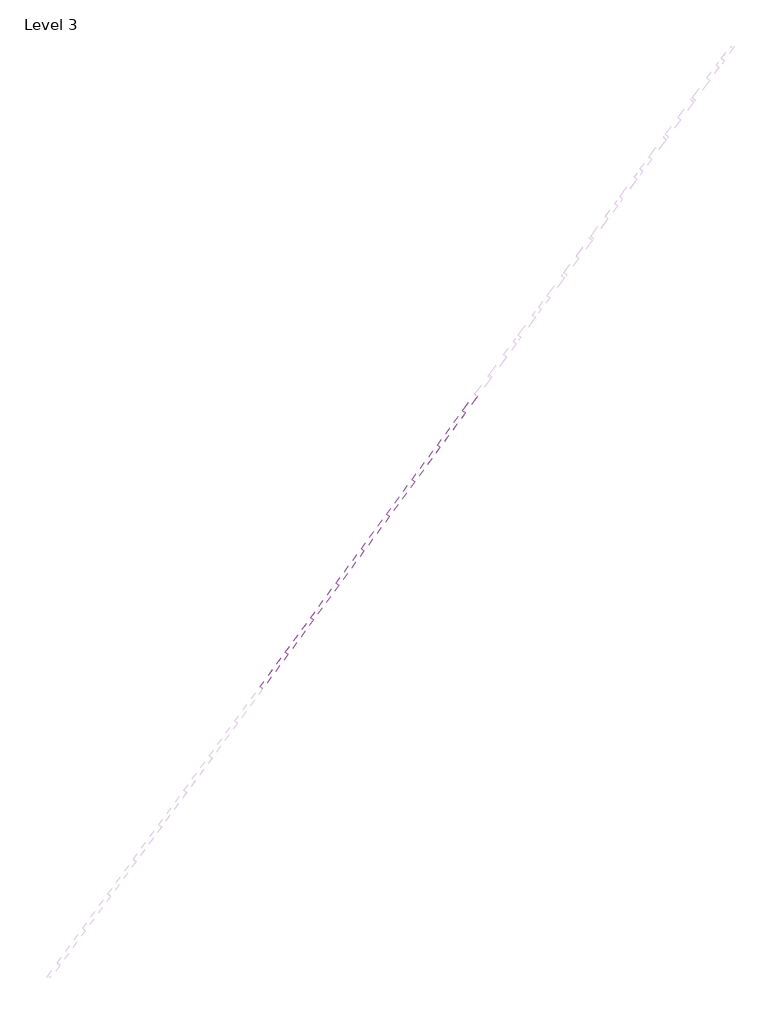
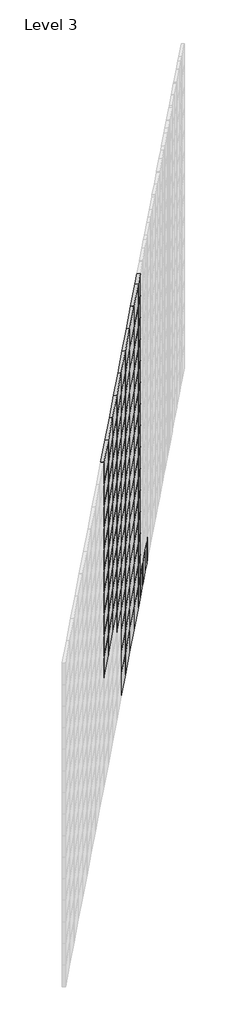
# One storey, part 3 of 9: 121 plates.
"""IFC4 building model written with IfcOpenShell, lengths in millimetres."""

import ifcopenshell
import ifcopenshell.guid

model = None  # the IFC model being written
_history = None  # IfcOwnerHistory: only IFC2X3 demands one
_inside = {}  # id of a spatial element -> (the spatial element, [elements in it])
_under = {}  # id of a project, library or spatial element -> (it, [spatial elements below it])
_declared = {}  # id of a project -> (the project, [libraries it declares])
_typed = {}  # id of a type object -> (the type object, [elements of that type])
_made_of = {}  # id of a material, layer set ... -> (it, [elements and type objects made of it])


def new_model(schema):
    """Start an empty IFC model of exactly this schema.

    Asked for "IFC4X3", IfcOpenShell would pick the latest addendum, in which some entities
    have other attributes; the version numbers below select the first issue.
    IFC2X3 requires an IfcOwnerHistory on every rooted entity: one is made here for all.
    """
    global model, _history
    if schema == "IFC4X3":
        model = ifcopenshell.file(schema_version=(4, 3, 0, 0))
    else:
        model = ifcopenshell.file(schema=schema)
    _inside.clear()
    _under.clear()
    _declared.clear()
    _typed.clear()
    _made_of.clear()
    _history = None
    if model.schema == "IFC2X3":
        org = make("IfcOrganization", Name="unknown")
        user = make(
            "IfcPersonAndOrganization",
            ThePerson=make("IfcPerson", FamilyName="unknown"),
            TheOrganization=org,
        )
        app = make(
            "IfcApplication",
            ApplicationDeveloper=org,
            Version="unknown",
            ApplicationFullName="unknown",
            ApplicationIdentifier="unknown",
        )
        _history = make(
            "IfcOwnerHistory",
            OwningUser=user,
            OwningApplication=app,
            ChangeAction="ADDED",
            CreationDate=0,
        )
    return model


def make(cls, **values):
    """One entity of the class cls with the attributes given. An attribute that is None is left unset."""
    return model.create_entity(
        cls, **{name: value for name, value in values.items() if value is not None}
    )


def rooted(cls, **values):
    """An entity with a GlobalId (a new one), such as an element, a storey or a relation."""
    return make(cls, GlobalId=ifcopenshell.guid.new(), OwnerHistory=_history, **values)


def si_unit(unit_type, name, prefix=None):
    """IfcSIUnit, for example si_unit("LENGTHUNIT", "METRE", prefix="MILLI")."""
    return make("IfcSIUnit", UnitType=unit_type, Prefix=prefix, Name=name)


def assignment(units):
    """IfcUnitAssignment: the units of a project."""
    return None if units is None else make("IfcUnitAssignment", Units=units)


def point(xyz):
    """IfcCartesianPoint."""
    return None if xyz is None else make("IfcCartesianPoint", Coordinates=xyz)


def direction(xyz):
    """IfcDirection."""
    return None if xyz is None else make("IfcDirection", DirectionRatios=xyz)


def frame(location, z_axis=None, x_axis=None):
    """IfcAxis2Placement3D, a coordinate frame: its origin and axes. An axis left out is left unset."""
    return make(
        "IfcAxis2Placement3D",
        Location=point(location),
        Axis=direction(z_axis),
        RefDirection=direction(x_axis),
    )


def origin():
    """The frame at (0, 0, 0) with its axes left unset."""
    return frame((0.0, 0.0, 0.0))


def origin_with_axes():
    """The frame at (0, 0, 0) with the z axis (0, 0, 1) and the x axis (1, 0, 0) written out."""
    return frame((0.0, 0.0, 0.0), z_axis=(0.0, 0.0, 1.0), x_axis=(1.0, 0.0, 0.0))


def place(relative_to, where):
    """IfcLocalPlacement: puts the frame where relative to a parent placement (None: the world)."""
    return make(
        "IfcLocalPlacement", PlacementRelTo=relative_to, RelativePlacement=where
    )


def context(
    kind, dimensions, precision=None, world=None, true_north=None, identifier=None
):
    """IfcGeometricRepresentationContext, for example the 3D "Model" context."""
    return make(
        "IfcGeometricRepresentationContext",
        ContextIdentifier=identifier,
        ContextType=kind,
        CoordinateSpaceDimension=dimensions,
        Precision=precision,
        WorldCoordinateSystem=world,
        TrueNorth=true_north,
    )


def project(units=None, contexts=None):
    """IfcProject with its units and contexts."""
    return rooted(
        "IfcProject",
        Name="project",
        RepresentationContexts=contexts,
        UnitsInContext=assignment(units),
    )


def spatial(cls, under=None, at=None, **own):
    """A site, building, storey or space (cls), placed at a placement, below another one or the project."""
    s = rooted(cls, ObjectPlacement=at, **own)
    if under is not None:
        _under.setdefault(under.id(), (under, []))[1].append(s)
    return s


def polyline(points):
    """IfcPolyline through the points."""
    return make("IfcPolyline", Points=[point(p) for p in points])


def outline(outer, holes=None, kind="AREA"):
    """IfcArbitraryClosedProfileDef: a profile drawn as a closed curve; with holes, ...WithVoids."""
    if holes is None:
        return make("IfcArbitraryClosedProfileDef", ProfileType=kind, OuterCurve=outer)
    return make(
        "IfcArbitraryProfileDefWithVoids",
        ProfileType=kind,
        OuterCurve=outer,
        InnerCurves=holes,
    )


def extrude(swept, where, along, depth):
    """IfcExtrudedAreaSolid: the profile swept, set in the frame where, extruded along a direction by depth."""
    return make(
        "IfcExtrudedAreaSolid",
        SweptArea=swept,
        Position=where,
        ExtrudedDirection=direction(along),
        Depth=depth,
    )


def shape(context_of_items, identifier, shape_type, items):
    """IfcShapeRepresentation: the items that make up one representation, for example the "Body"."""
    return make(
        "IfcShapeRepresentation",
        ContextOfItems=context_of_items,
        RepresentationIdentifier=identifier,
        RepresentationType=shape_type,
        Items=items,
    )


def source(mapping_origin, context_of_items, identifier, shape_type, items):
    """IfcRepresentationMap: a shape defined once, which mapped items show again and again."""
    return make(
        "IfcRepresentationMap",
        MappingOrigin=mapping_origin,
        MappedRepresentation=shape(context_of_items, identifier, shape_type, items),
    )


def transform(
    local_origin,
    x_axis=None,
    y_axis=None,
    z_axis=None,
    scale=None,
    scale2=None,
    scale3=None,
    uniform=True,
):
    """IfcCartesianTransformationOperator3D, or its non-uniform kind. x_axis, y_axis, z_axis: its Axis1, 2, 3."""
    if uniform:
        return make(
            "IfcCartesianTransformationOperator3D",
            Axis1=direction(x_axis),
            Axis2=direction(y_axis),
            LocalOrigin=point(local_origin),
            Scale=scale,
            Axis3=direction(z_axis),
        )
    return make(
        "IfcCartesianTransformationOperator3DnonUniform",
        Axis1=direction(x_axis),
        Axis2=direction(y_axis),
        LocalOrigin=point(local_origin),
        Scale=scale,
        Axis3=direction(z_axis),
        Scale2=scale2,
        Scale3=scale3,
    )


def mapped(mapping_source, mapping_target):
    """IfcMappedItem: shows the shape of a source again, moved by a transform."""
    return make(
        "IfcMappedItem", MappingSource=mapping_source, MappingTarget=mapping_target
    )


def made_of(thing, what):
    """Note that an element or type object is made of a material, layer set ...; save() writes the relation."""
    if what is not None:
        _made_of.setdefault(what.id(), (what, []))[1].append(thing)
    return thing


def element(
    cls,
    number,
    at=None,
    inside=None,
    cuts=None,
    type_object=None,
    material=None,
    context=None,
    identifier="Body",
    shape_type=None,
    held_by="IfcProductDefinitionShape",
    body=None,
    shapes=None,
    **own,
):
    """One element of the class cls, such as IfcWall. Its Tag is "e" and its number.

    at: its placement. inside: the storey or other place that contains it. cuts: it is an
    opening in that element (IfcRelVoidsElement). A single representation is given by context,
    identifier, shape_type and body (its items); several are given by shapes. held_by: the class
    of the entity that holds the representations. save() writes the other relations.
    """
    e = rooted(cls, Tag="e%d" % number, ObjectPlacement=at, **own)
    if body is not None:
        shapes = [shape(context, identifier, shape_type, body)]
    if shapes is not None:
        e.Representation = make(held_by, Representations=shapes)
    if inside is not None:
        _inside.setdefault(inside.id(), (inside, []))[1].append(e)
    if cuts is not None:
        rooted(
            "IfcRelVoidsElement", RelatingBuildingElement=cuts, RelatedOpeningElement=e
        )
    if type_object is not None:
        _typed.setdefault(type_object.id(), (type_object, []))[1].append(e)
    return made_of(e, material)


def aggregate(whole, parts):
    """IfcRelAggregates: a whole, such as a stair, and the parts it consists of."""
    return rooted("IfcRelAggregates", RelatingObject=whole, RelatedObjects=parts)


def save(model, path):
    """Write the relations noted so far, then the file.

    IfcRelAggregates (storeys below a building ...), IfcRelContainedInSpatialStructure (elements
    in a storey), IfcRelDefinesByType, IfcRelAssociatesMaterial and IfcRelDeclares: one each for
    every whole, place, type object, material and project.
    """
    for whole, parts in _under.values():
        aggregate(whole, parts)
    for where, things in _inside.values():
        rooted(
            "IfcRelContainedInSpatialStructure",
            RelatedElements=things,
            RelatingStructure=where,
        )
    for kind, things in _typed.values():
        rooted("IfcRelDefinesByType", RelatedObjects=things, RelatingType=kind)
    for what, things in _made_of.values():
        rooted("IfcRelAssociatesMaterial", RelatedObjects=things, RelatingMaterial=what)
    for by, libraries in _declared.values():
        rooted("IfcRelDeclares", RelatingContext=by, RelatedDefinitions=libraries)
    model.write(path)


def system_panel_glazed_2fc8f5ca(model_context):
    return source(origin(), model_context, "Body", "SweptSolid", [
        extrude(outline(polyline([(148.4832393, 24.5), (-148.4832393, 24.5), (-148.4832393, 49.5), (148.4832393, 49.5), (148.4832393, 24.5)])), origin_with_axes(), (0.0, 0.0, 1.0), 200.0),
    ])


def system_panel_glazed_b673c039(model_context):
    return source(origin(), model_context, "Body", "SweptSolid", [
        extrude(outline(polyline([(69.8854993, 24.5), (-69.8854993, 24.5), (-69.8854993, 49.5), (69.8854993, 49.5), (69.8854993, 24.5)])), origin_with_axes(), (0.0, 0.0, 1.0), 200.0),
    ])


def system_panel_glazed_de35cd91(model_context):
    return source(origin(), model_context, "Body", "SweptSolid", [
        extrude(outline(polyline([(6.4022601, 24.5), (-6.4022601, 24.5), (-6.4022601, 49.5), (6.4022601, 49.5), (6.4022601, 24.5)])), origin_with_axes(), (0.0, 0.0, 1.0), 200.0),
    ])


def system_panel_glazed_77252c6e(model_context):
    return source(origin(), model_context, "Body", "SweptSolid", [
        extrude(outline(polyline([(27.919021, 24.5), (-27.919021, 24.5), (-27.919021, 49.5), (27.919021, 49.5), (27.919021, 24.5)])), origin_with_axes(), (0.0, 0.0, 1.0), 200.0),
    ])


def system_panel_glazed_165eaad2(model_context):
    return source(origin(), model_context, "Body", "SweptSolid", [
        extrude(outline(polyline([(78.5977399, 24.5), (-78.5977399, 24.5), (-78.5977399, 49.5), (78.5977399, 49.5), (78.5977399, 24.5)])), origin_with_axes(), (0.0, 0.0, 1.0), 200.0),
    ])


def system_panel_glazed_1ea8d406(model_context):
    return source(origin(), model_context, "Body", "SweptSolid", [
        extrude(outline(polyline([(85.0, 24.5), (-85.0, 24.5), (-85.0, 49.5), (85.0, 49.5), (85.0, 24.5)])), origin_with_axes(), (0.0, 0.0, 1.0), 200.0),
    ])


def system_panel_glazed_41e93d41(model_context):
    return source(origin(), model_context, "Body", "SweptSolid", [
        extrude(outline(polyline([(57.080979, 24.5), (-57.080979, 24.5), (-57.080979, 49.5), (57.080979, 49.5), (57.080979, 24.5)])), origin_with_axes(), (0.0, 0.0, 1.0), 200.0),
    ])


model = new_model("IFC4")

# Units and contexts
model_context = context("Model", 3, world=origin())
ifc_project = project(units=[si_unit("LENGTHUNIT", "METRE", prefix="MILLI")], contexts=[model_context])

# Site, building, storey
site = spatial("IfcSite", under=ifc_project)
building = spatial("IfcBuilding", under=site)
storey = spatial("IfcBuildingStorey", under=building, Name="Level 3", Elevation=22950.0)

# Plates
placement = place(None, origin())
system_panel_glazed_shape = system_panel_glazed_2fc8f5ca(model_context)
element("IfcPlate", 1, ObjectType="System Panel : Glazed", at=placement, inside=storey, context=model_context, shape_type="MappedRepresentation", body=[
    mapped(system_panel_glazed_shape, transform((-34075.7749604, 27069.7374952, 35100.0), x_axis=(0.5920548138930122, 0.8058976965757569, 0.0), y_axis=(-0.8058976965757569, 0.5920548138930122, 0.0), z_axis=(0.0, 0.0, 1.0))),
])
element("IfcPlate", 2, ObjectType="System Panel : Glazed", at=placement, inside=storey, context=model_context, shape_type="MappedRepresentation", body=[
    mapped(system_panel_glazed_shape, transform((-33899.9545274, 27309.0620961, 35100.0), x_axis=(0.5920548138930122, 0.8058976965757569, 0.0), y_axis=(-0.8058976965757569, 0.5920548138930122, 0.0), z_axis=(0.0, 0.0, 1.0))),
])
element("IfcPlate", 3, ObjectType="System Panel : Glazed", at=placement, inside=storey, context=model_context, shape_type="MappedRepresentation", body=[
    mapped(system_panel_glazed_shape, transform((-33724.1340943, 27548.3866969, 35100.0), x_axis=(0.5920548138930122, 0.8058976965757569, 0.0), y_axis=(-0.8058976965757569, 0.5920548138930122, 0.0), z_axis=(0.0, 0.0, 1.0))),
])
element("IfcPlate", 4, ObjectType="System Panel : Glazed", at=placement, inside=storey, context=model_context, shape_type="MappedRepresentation", body=[
    mapped(system_panel_glazed_shape, transform((-33548.3136613, 27787.7112977, 35100.0), x_axis=(0.5920548138930122, 0.8058976965757569, 0.0), y_axis=(-0.8058976965757569, 0.5920548138930122, 0.0), z_axis=(0.0, 0.0, 1.0))),
])
element("IfcPlate", 5, ObjectType="System Panel : Glazed", at=placement, inside=storey, context=model_context, shape_type="MappedRepresentation", body=[
    mapped(system_panel_glazed_shape, transform((-34075.7749604, 27069.7374952, 35300.0), x_axis=(0.5920548138930122, 0.8058976965757569, 0.0), y_axis=(-0.8058976965757569, 0.5920548138930122, 0.0), z_axis=(0.0, 0.0, 1.0))),
])
element("IfcPlate", 6, ObjectType="System Panel : Glazed", at=placement, inside=storey, context=model_context, shape_type="MappedRepresentation", body=[
    mapped(system_panel_glazed_shape, transform((-33899.9545274, 27309.0620961, 35300.0), x_axis=(0.5920548138930122, 0.8058976965757569, 0.0), y_axis=(-0.8058976965757569, 0.5920548138930122, 0.0), z_axis=(0.0, 0.0, 1.0))),
])
element("IfcPlate", 7, ObjectType="System Panel : Glazed", at=placement, inside=storey, context=model_context, shape_type="MappedRepresentation", body=[
    mapped(system_panel_glazed_shape, transform((-33724.1340943, 27548.3866969, 35300.0), x_axis=(0.5920548138930122, 0.8058976965757569, 0.0), y_axis=(-0.8058976965757569, 0.5920548138930122, 0.0), z_axis=(0.0, 0.0, 1.0))),
])
element("IfcPlate", 8, ObjectType="System Panel : Glazed", at=placement, inside=storey, context=model_context, shape_type="MappedRepresentation", body=[
    mapped(system_panel_glazed_shape, transform((-33548.3136613, 27787.7112977, 35300.0), x_axis=(0.5920548138930122, 0.8058976965757569, 0.0), y_axis=(-0.8058976965757569, 0.5920548138930122, 0.0), z_axis=(0.0, 0.0, 1.0))),
])
element("IfcPlate", 9, ObjectType="System Panel : Glazed", at=placement, inside=storey, context=model_context, shape_type="MappedRepresentation", body=[
    mapped(system_panel_glazed_shape, transform((-34075.7749604, 27069.7374952, 35500.0), x_axis=(0.5920548138930122, 0.8058976965757569, 0.0), y_axis=(-0.8058976965757569, 0.5920548138930122, 0.0), z_axis=(0.0, 0.0, 1.0))),
])
element("IfcPlate", 10, ObjectType="System Panel : Glazed", at=placement, inside=storey, context=model_context, shape_type="MappedRepresentation", body=[
    mapped(system_panel_glazed_shape, transform((-33899.9545274, 27309.0620961, 35500.0), x_axis=(0.5920548138930122, 0.8058976965757569, 0.0), y_axis=(-0.8058976965757569, 0.5920548138930122, 0.0), z_axis=(0.0, 0.0, 1.0))),
])
element("IfcPlate", 11, ObjectType="System Panel : Glazed", at=placement, inside=storey, context=model_context, shape_type="MappedRepresentation", body=[
    mapped(system_panel_glazed_shape, transform((-33724.1340943, 27548.3866969, 35500.0), x_axis=(0.5920548138930122, 0.8058976965757569, 0.0), y_axis=(-0.8058976965757569, 0.5920548138930122, 0.0), z_axis=(0.0, 0.0, 1.0))),
])
element("IfcPlate", 12, ObjectType="System Panel : Glazed", at=placement, inside=storey, context=model_context, shape_type="MappedRepresentation", body=[
    mapped(system_panel_glazed_shape, transform((-33548.3136613, 27787.7112977, 35500.0), x_axis=(0.5920548138930122, 0.8058976965757569, 0.0), y_axis=(-0.8058976965757569, 0.5920548138930122, 0.0), z_axis=(0.0, 0.0, 1.0))),
])
element("IfcPlate", 13, ObjectType="System Panel : Glazed", at=placement, inside=storey, context=model_context, shape_type="MappedRepresentation", body=[
    mapped(system_panel_glazed_shape, transform((-34075.7749604, 27069.7374952, 35700.0), x_axis=(0.5920548138930122, 0.8058976965757569, 0.0), y_axis=(-0.8058976965757569, 0.5920548138930122, 0.0), z_axis=(0.0, 0.0, 1.0))),
])
element("IfcPlate", 14, ObjectType="System Panel : Glazed", at=placement, inside=storey, context=model_context, shape_type="MappedRepresentation", body=[
    mapped(system_panel_glazed_shape, transform((-33899.9545274, 27309.0620961, 35700.0), x_axis=(0.5920548138930122, 0.8058976965757569, 0.0), y_axis=(-0.8058976965757569, 0.5920548138930122, 0.0), z_axis=(0.0, 0.0, 1.0))),
])
element("IfcPlate", 15, ObjectType="System Panel : Glazed", at=placement, inside=storey, context=model_context, shape_type="MappedRepresentation", body=[
    mapped(system_panel_glazed_shape, transform((-33724.1340943, 27548.3866969, 35700.0), x_axis=(0.5920548138930122, 0.8058976965757569, 0.0), y_axis=(-0.8058976965757569, 0.5920548138930122, 0.0), z_axis=(0.0, 0.0, 1.0))),
])
element("IfcPlate", 16, ObjectType="System Panel : Glazed", at=placement, inside=storey, context=model_context, shape_type="MappedRepresentation", body=[
    mapped(system_panel_glazed_shape, transform((-33548.3136613, 27787.7112977, 35700.0), x_axis=(0.5920548138930122, 0.8058976965757569, 0.0), y_axis=(-0.8058976965757569, 0.5920548138930122, 0.0), z_axis=(0.0, 0.0, 1.0))),
])
element("IfcPlate", 17, ObjectType="System Panel : Glazed", at=placement, inside=storey, context=model_context, shape_type="MappedRepresentation", body=[
    mapped(system_panel_glazed_shape, transform((-34251.5953935, 26830.4128944, 35900.0), x_axis=(0.5920548138930122, 0.8058976965757569, 0.0), y_axis=(-0.8058976965757569, 0.5920548138930122, 0.0), z_axis=(0.0, 0.0, 1.0))),
])
element("IfcPlate", 18, ObjectType="System Panel : Glazed", at=placement, inside=storey, context=model_context, shape_type="MappedRepresentation", body=[
    mapped(system_panel_glazed_shape, transform((-34075.7749604, 27069.7374952, 35900.0), x_axis=(0.5920548138930122, 0.8058976965757569, 0.0), y_axis=(-0.8058976965757569, 0.5920548138930122, 0.0), z_axis=(0.0, 0.0, 1.0))),
])
element("IfcPlate", 19, ObjectType="System Panel : Glazed", at=placement, inside=storey, context=model_context, shape_type="MappedRepresentation", body=[
    mapped(system_panel_glazed_shape, transform((-33899.9545274, 27309.0620961, 35900.0), x_axis=(0.5920548138930122, 0.8058976965757569, 0.0), y_axis=(-0.8058976965757569, 0.5920548138930122, 0.0), z_axis=(0.0, 0.0, 1.0))),
])
element("IfcPlate", 20, ObjectType="System Panel : Glazed", at=placement, inside=storey, context=model_context, shape_type="MappedRepresentation", body=[
    mapped(system_panel_glazed_shape, transform((-33724.1340943, 27548.3866969, 35900.0), x_axis=(0.5920548138930122, 0.8058976965757569, 0.0), y_axis=(-0.8058976965757569, 0.5920548138930122, 0.0), z_axis=(0.0, 0.0, 1.0))),
])
element("IfcPlate", 21, ObjectType="System Panel : Glazed", at=placement, inside=storey, context=model_context, shape_type="MappedRepresentation", body=[
    mapped(system_panel_glazed_shape, transform((-33548.3136613, 27787.7112977, 35900.0), x_axis=(0.5920548138930122, 0.8058976965757569, 0.0), y_axis=(-0.8058976965757569, 0.5920548138930122, 0.0), z_axis=(0.0, 0.0, 1.0))),
])
element("IfcPlate", 22, ObjectType="System Panel : Glazed", at=placement, inside=storey, context=model_context, shape_type="MappedRepresentation", body=[
    mapped(system_panel_glazed_shape, transform((-34779.0566927, 26112.4390918, 36100.0), x_axis=(0.5920548138930122, 0.8058976965757569, 0.0), y_axis=(-0.8058976965757569, 0.5920548138930122, 0.0), z_axis=(0.0, 0.0, 1.0))),
])
element("IfcPlate", 23, ObjectType="System Panel : Glazed", at=placement, inside=storey, context=model_context, shape_type="MappedRepresentation", body=[
    mapped(system_panel_glazed_shape, transform((-34603.2362596, 26351.7636927, 36100.0), x_axis=(0.5920548138930122, 0.8058976965757569, 0.0), y_axis=(-0.8058976965757569, 0.5920548138930122, 0.0), z_axis=(0.0, 0.0, 1.0))),
])
element("IfcPlate", 24, ObjectType="System Panel : Glazed", at=placement, inside=storey, context=model_context, shape_type="MappedRepresentation", body=[
    mapped(system_panel_glazed_shape, transform((-34427.4158266, 26591.0882935, 36100.0), x_axis=(0.5920548138930122, 0.8058976965757569, 0.0), y_axis=(-0.8058976965757569, 0.5920548138930122, 0.0), z_axis=(0.0, 0.0, 1.0))),
])
element("IfcPlate", 25, ObjectType="System Panel : Glazed", at=placement, inside=storey, context=model_context, shape_type="MappedRepresentation", body=[
    mapped(system_panel_glazed_shape, transform((-34251.5953935, 26830.4128944, 36100.0), x_axis=(0.5920548138930122, 0.8058976965757569, 0.0), y_axis=(-0.8058976965757569, 0.5920548138930122, 0.0), z_axis=(0.0, 0.0, 1.0))),
])
element("IfcPlate", 26, ObjectType="System Panel : Glazed", at=placement, inside=storey, context=model_context, shape_type="MappedRepresentation", body=[
    mapped(system_panel_glazed_shape, transform((-34075.7749604, 27069.7374952, 36100.0), x_axis=(0.5920548138930122, 0.8058976965757569, 0.0), y_axis=(-0.8058976965757569, 0.5920548138930122, 0.0), z_axis=(0.0, 0.0, 1.0))),
])
element("IfcPlate", 27, ObjectType="System Panel : Glazed", at=placement, inside=storey, context=model_context, shape_type="MappedRepresentation", body=[
    mapped(system_panel_glazed_shape, transform((-33899.9545274, 27309.0620961, 36100.0), x_axis=(0.5920548138930122, 0.8058976965757569, 0.0), y_axis=(-0.8058976965757569, 0.5920548138930122, 0.0), z_axis=(0.0, 0.0, 1.0))),
])
element("IfcPlate", 28, ObjectType="System Panel : Glazed", at=placement, inside=storey, context=model_context, shape_type="MappedRepresentation", body=[
    mapped(system_panel_glazed_shape, transform((-33724.1340943, 27548.3866969, 36100.0), x_axis=(0.5920548138930122, 0.8058976965757569, 0.0), y_axis=(-0.8058976965757569, 0.5920548138930122, 0.0), z_axis=(0.0, 0.0, 1.0))),
])
element("IfcPlate", 29, ObjectType="System Panel : Glazed", at=placement, inside=storey, context=model_context, shape_type="MappedRepresentation", body=[
    mapped(system_panel_glazed_shape, transform((-33548.3136613, 27787.7112977, 36100.0), x_axis=(0.5920548138930122, 0.8058976965757569, 0.0), y_axis=(-0.8058976965757569, 0.5920548138930122, 0.0), z_axis=(0.0, 0.0, 1.0))),
])
element("IfcPlate", 30, ObjectType="System Panel : Glazed", at=placement, inside=storey, context=model_context, shape_type="MappedRepresentation", body=[
    mapped(system_panel_glazed_shape, transform((-34779.0566927, 26112.4390918, 36300.0), x_axis=(0.5920548138930122, 0.8058976965757569, 0.0), y_axis=(-0.8058976965757569, 0.5920548138930122, 0.0), z_axis=(0.0, 0.0, 1.0))),
])
element("IfcPlate", 31, ObjectType="System Panel : Glazed", at=placement, inside=storey, context=model_context, shape_type="MappedRepresentation", body=[
    mapped(system_panel_glazed_shape, transform((-34603.2362596, 26351.7636927, 36300.0), x_axis=(0.5920548138930122, 0.8058976965757569, 0.0), y_axis=(-0.8058976965757569, 0.5920548138930122, 0.0), z_axis=(0.0, 0.0, 1.0))),
])
element("IfcPlate", 32, ObjectType="System Panel : Glazed", at=placement, inside=storey, context=model_context, shape_type="MappedRepresentation", body=[
    mapped(system_panel_glazed_shape, transform((-34427.4158266, 26591.0882935, 36300.0), x_axis=(0.5920548138930122, 0.8058976965757569, 0.0), y_axis=(-0.8058976965757569, 0.5920548138930122, 0.0), z_axis=(0.0, 0.0, 1.0))),
])
element("IfcPlate", 33, ObjectType="System Panel : Glazed", at=placement, inside=storey, context=model_context, shape_type="MappedRepresentation", body=[
    mapped(system_panel_glazed_shape, transform((-34251.5953935, 26830.4128944, 36300.0), x_axis=(0.5920548138930122, 0.8058976965757569, 0.0), y_axis=(-0.8058976965757569, 0.5920548138930122, 0.0), z_axis=(0.0, 0.0, 1.0))),
])
element("IfcPlate", 34, ObjectType="System Panel : Glazed", at=placement, inside=storey, context=model_context, shape_type="MappedRepresentation", body=[
    mapped(system_panel_glazed_shape, transform((-34075.7749604, 27069.7374952, 36300.0), x_axis=(0.5920548138930122, 0.8058976965757569, 0.0), y_axis=(-0.8058976965757569, 0.5920548138930122, 0.0), z_axis=(0.0, 0.0, 1.0))),
])
element("IfcPlate", 35, ObjectType="System Panel : Glazed", at=placement, inside=storey, context=model_context, shape_type="MappedRepresentation", body=[
    mapped(system_panel_glazed_shape, transform((-33899.9545274, 27309.0620961, 36300.0), x_axis=(0.5920548138930122, 0.8058976965757569, 0.0), y_axis=(-0.8058976965757569, 0.5920548138930122, 0.0), z_axis=(0.0, 0.0, 1.0))),
])
element("IfcPlate", 36, ObjectType="System Panel : Glazed", at=placement, inside=storey, context=model_context, shape_type="MappedRepresentation", body=[
    mapped(system_panel_glazed_shape, transform((-33724.1340943, 27548.3866969, 36300.0), x_axis=(0.5920548138930122, 0.8058976965757569, 0.0), y_axis=(-0.8058976965757569, 0.5920548138930122, 0.0), z_axis=(0.0, 0.0, 1.0))),
])
element("IfcPlate", 37, ObjectType="System Panel : Glazed", at=placement, inside=storey, context=model_context, shape_type="MappedRepresentation", body=[
    mapped(system_panel_glazed_shape, transform((-33548.3136613, 27787.7112977, 36300.0), x_axis=(0.5920548138930122, 0.8058976965757569, 0.0), y_axis=(-0.8058976965757569, 0.5920548138930122, 0.0), z_axis=(0.0, 0.0, 1.0))),
])
element("IfcPlate", 38, ObjectType="System Panel : Glazed", at=placement, inside=storey, context=model_context, shape_type="MappedRepresentation", body=[
    mapped(system_panel_glazed_shape, transform((-34779.0566927, 26112.4390918, 36500.0), x_axis=(0.5920548138930122, 0.8058976965757569, 0.0), y_axis=(-0.8058976965757569, 0.5920548138930122, 0.0), z_axis=(0.0, 0.0, 1.0))),
])
element("IfcPlate", 39, ObjectType="System Panel : Glazed", at=placement, inside=storey, context=model_context, shape_type="MappedRepresentation", body=[
    mapped(system_panel_glazed_shape, transform((-34603.2362596, 26351.7636927, 36500.0), x_axis=(0.5920548138930122, 0.8058976965757569, 0.0), y_axis=(-0.8058976965757569, 0.5920548138930122, 0.0), z_axis=(0.0, 0.0, 1.0))),
])
element("IfcPlate", 40, ObjectType="System Panel : Glazed", at=placement, inside=storey, context=model_context, shape_type="MappedRepresentation", body=[
    mapped(system_panel_glazed_shape, transform((-34427.4158266, 26591.0882935, 36500.0), x_axis=(0.5920548138930122, 0.8058976965757569, 0.0), y_axis=(-0.8058976965757569, 0.5920548138930122, 0.0), z_axis=(0.0, 0.0, 1.0))),
])
element("IfcPlate", 41, ObjectType="System Panel : Glazed", at=placement, inside=storey, context=model_context, shape_type="MappedRepresentation", body=[
    mapped(system_panel_glazed_shape, transform((-34251.5953935, 26830.4128944, 36500.0), x_axis=(0.5920548138930122, 0.8058976965757569, 0.0), y_axis=(-0.8058976965757569, 0.5920548138930122, 0.0), z_axis=(0.0, 0.0, 1.0))),
])
element("IfcPlate", 42, ObjectType="System Panel : Glazed", at=placement, inside=storey, context=model_context, shape_type="MappedRepresentation", body=[
    mapped(system_panel_glazed_shape, transform((-34075.7749604, 27069.7374952, 36500.0), x_axis=(0.5920548138930122, 0.8058976965757569, 0.0), y_axis=(-0.8058976965757569, 0.5920548138930122, 0.0), z_axis=(0.0, 0.0, 1.0))),
])
element("IfcPlate", 43, ObjectType="System Panel : Glazed", at=placement, inside=storey, context=model_context, shape_type="MappedRepresentation", body=[
    mapped(system_panel_glazed_shape, transform((-33899.9545274, 27309.0620961, 36500.0), x_axis=(0.5920548138930122, 0.8058976965757569, 0.0), y_axis=(-0.8058976965757569, 0.5920548138930122, 0.0), z_axis=(0.0, 0.0, 1.0))),
])
element("IfcPlate", 44, ObjectType="System Panel : Glazed", at=placement, inside=storey, context=model_context, shape_type="MappedRepresentation", body=[
    mapped(system_panel_glazed_shape, transform((-33724.1340943, 27548.3866969, 36500.0), x_axis=(0.5920548138930122, 0.8058976965757569, 0.0), y_axis=(-0.8058976965757569, 0.5920548138930122, 0.0), z_axis=(0.0, 0.0, 1.0))),
])
element("IfcPlate", 45, ObjectType="System Panel : Glazed", at=placement, inside=storey, context=model_context, shape_type="MappedRepresentation", body=[
    mapped(system_panel_glazed_shape, transform((-33548.3136613, 27787.7112977, 36500.0), x_axis=(0.5920548138930122, 0.8058976965757569, 0.0), y_axis=(-0.8058976965757569, 0.5920548138930122, 0.0), z_axis=(0.0, 0.0, 1.0))),
])
element("IfcPlate", 46, ObjectType="System Panel : Glazed", at=placement, inside=storey, context=model_context, shape_type="MappedRepresentation", body=[
    mapped(system_panel_glazed_shape, transform((-34779.0566927, 26112.4390918, 36700.0), x_axis=(0.5920548138930122, 0.8058976965757569, 0.0), y_axis=(-0.8058976965757569, 0.5920548138930122, 0.0), z_axis=(0.0, 0.0, 1.0))),
])
element("IfcPlate", 47, ObjectType="System Panel : Glazed", at=placement, inside=storey, context=model_context, shape_type="MappedRepresentation", body=[
    mapped(system_panel_glazed_shape, transform((-34603.2362596, 26351.7636927, 36700.0), x_axis=(0.5920548138930122, 0.8058976965757569, 0.0), y_axis=(-0.8058976965757569, 0.5920548138930122, 0.0), z_axis=(0.0, 0.0, 1.0))),
])
element("IfcPlate", 48, ObjectType="System Panel : Glazed", at=placement, inside=storey, context=model_context, shape_type="MappedRepresentation", body=[
    mapped(system_panel_glazed_shape, transform((-34427.4158266, 26591.0882935, 36700.0), x_axis=(0.5920548138930122, 0.8058976965757569, 0.0), y_axis=(-0.8058976965757569, 0.5920548138930122, 0.0), z_axis=(0.0, 0.0, 1.0))),
])
element("IfcPlate", 49, ObjectType="System Panel : Glazed", at=placement, inside=storey, context=model_context, shape_type="MappedRepresentation", body=[
    mapped(system_panel_glazed_shape, transform((-34251.5953935, 26830.4128944, 36700.0), x_axis=(0.5920548138930122, 0.8058976965757569, 0.0), y_axis=(-0.8058976965757569, 0.5920548138930122, 0.0), z_axis=(0.0, 0.0, 1.0))),
])
element("IfcPlate", 50, ObjectType="System Panel : Glazed", at=placement, inside=storey, context=model_context, shape_type="MappedRepresentation", body=[
    mapped(system_panel_glazed_shape, transform((-34075.7749604, 27069.7374952, 36700.0), x_axis=(0.5920548138930122, 0.8058976965757569, 0.0), y_axis=(-0.8058976965757569, 0.5920548138930122, 0.0), z_axis=(0.0, 0.0, 1.0))),
])
element("IfcPlate", 51, ObjectType="System Panel : Glazed", at=placement, inside=storey, context=model_context, shape_type="MappedRepresentation", body=[
    mapped(system_panel_glazed_shape, transform((-33899.9545274, 27309.0620961, 36700.0), x_axis=(0.5920548138930122, 0.8058976965757569, 0.0), y_axis=(-0.8058976965757569, 0.5920548138930122, 0.0), z_axis=(0.0, 0.0, 1.0))),
])
element("IfcPlate", 52, ObjectType="System Panel : Glazed", at=placement, inside=storey, context=model_context, shape_type="MappedRepresentation", body=[
    mapped(system_panel_glazed_shape, transform((-33724.1340943, 27548.3866969, 36700.0), x_axis=(0.5920548138930122, 0.8058976965757569, 0.0), y_axis=(-0.8058976965757569, 0.5920548138930122, 0.0), z_axis=(0.0, 0.0, 1.0))),
])
element("IfcPlate", 53, ObjectType="System Panel : Glazed", at=placement, inside=storey, context=model_context, shape_type="MappedRepresentation", body=[
    mapped(system_panel_glazed_shape, transform((-33548.3136613, 27787.7112977, 36700.0), x_axis=(0.5920548138930122, 0.8058976965757569, 0.0), y_axis=(-0.8058976965757569, 0.5920548138930122, 0.0), z_axis=(0.0, 0.0, 1.0))),
])
element("IfcPlate", 54, ObjectType="System Panel : Glazed", at=placement, inside=storey, context=model_context, shape_type="MappedRepresentation", body=[
    mapped(system_panel_glazed_shape, transform((-34779.0566927, 26112.4390918, 36900.0), x_axis=(0.5920548138930122, 0.8058976965757569, 0.0), y_axis=(-0.8058976965757569, 0.5920548138930122, 0.0), z_axis=(0.0, 0.0, 1.0))),
])
element("IfcPlate", 55, ObjectType="System Panel : Glazed", at=placement, inside=storey, context=model_context, shape_type="MappedRepresentation", body=[
    mapped(system_panel_glazed_shape, transform((-34603.2362596, 26351.7636927, 36900.0), x_axis=(0.5920548138930122, 0.8058976965757569, 0.0), y_axis=(-0.8058976965757569, 0.5920548138930122, 0.0), z_axis=(0.0, 0.0, 1.0))),
])
element("IfcPlate", 56, ObjectType="System Panel : Glazed", at=placement, inside=storey, context=model_context, shape_type="MappedRepresentation", body=[
    mapped(system_panel_glazed_shape, transform((-34427.4158266, 26591.0882935, 36900.0), x_axis=(0.5920548138930122, 0.8058976965757569, 0.0), y_axis=(-0.8058976965757569, 0.5920548138930122, 0.0), z_axis=(0.0, 0.0, 1.0))),
])
element("IfcPlate", 57, ObjectType="System Panel : Glazed", at=placement, inside=storey, context=model_context, shape_type="MappedRepresentation", body=[
    mapped(system_panel_glazed_shape, transform((-34251.5953935, 26830.4128944, 36900.0), x_axis=(0.5920548138930122, 0.8058976965757569, 0.0), y_axis=(-0.8058976965757569, 0.5920548138930122, 0.0), z_axis=(0.0, 0.0, 1.0))),
])
element("IfcPlate", 58, ObjectType="System Panel : Glazed", at=placement, inside=storey, context=model_context, shape_type="MappedRepresentation", body=[
    mapped(system_panel_glazed_shape, transform((-34075.7749604, 27069.7374952, 36900.0), x_axis=(0.5920548138930122, 0.8058976965757569, 0.0), y_axis=(-0.8058976965757569, 0.5920548138930122, 0.0), z_axis=(0.0, 0.0, 1.0))),
])
element("IfcPlate", 59, ObjectType="System Panel : Glazed", at=placement, inside=storey, context=model_context, shape_type="MappedRepresentation", body=[
    mapped(system_panel_glazed_shape, transform((-33899.9545274, 27309.0620961, 36900.0), x_axis=(0.5920548138930122, 0.8058976965757569, 0.0), y_axis=(-0.8058976965757569, 0.5920548138930122, 0.0), z_axis=(0.0, 0.0, 1.0))),
])
element("IfcPlate", 60, ObjectType="System Panel : Glazed", at=placement, inside=storey, context=model_context, shape_type="MappedRepresentation", body=[
    mapped(system_panel_glazed_shape, transform((-33724.1340943, 27548.3866969, 36900.0), x_axis=(0.5920548138930122, 0.8058976965757569, 0.0), y_axis=(-0.8058976965757569, 0.5920548138930122, 0.0), z_axis=(0.0, 0.0, 1.0))),
])
element("IfcPlate", 61, ObjectType="System Panel : Glazed", at=placement, inside=storey, context=model_context, shape_type="MappedRepresentation", body=[
    mapped(system_panel_glazed_shape, transform((-33548.3136613, 27787.7112977, 36900.0), x_axis=(0.5920548138930122, 0.8058976965757569, 0.0), y_axis=(-0.8058976965757569, 0.5920548138930122, 0.0), z_axis=(0.0, 0.0, 1.0))),
])
element("IfcPlate", 62, ObjectType="System Panel : Glazed", at=placement, inside=storey, context=model_context, shape_type="MappedRepresentation", body=[
    mapped(system_panel_glazed_shape, transform((-34779.0566927, 26112.4390918, 37100.0), x_axis=(0.5920548138930122, 0.8058976965757569, 0.0), y_axis=(-0.8058976965757569, 0.5920548138930122, 0.0), z_axis=(0.0, 0.0, 1.0))),
])
element("IfcPlate", 63, ObjectType="System Panel : Glazed", at=placement, inside=storey, context=model_context, shape_type="MappedRepresentation", body=[
    mapped(system_panel_glazed_shape, transform((-34603.2362596, 26351.7636927, 37100.0), x_axis=(0.5920548138930122, 0.8058976965757569, 0.0), y_axis=(-0.8058976965757569, 0.5920548138930122, 0.0), z_axis=(0.0, 0.0, 1.0))),
])
element("IfcPlate", 64, ObjectType="System Panel : Glazed", at=placement, inside=storey, context=model_context, shape_type="MappedRepresentation", body=[
    mapped(system_panel_glazed_shape, transform((-34427.4158266, 26591.0882935, 37100.0), x_axis=(0.5920548138930122, 0.8058976965757569, 0.0), y_axis=(-0.8058976965757569, 0.5920548138930122, 0.0), z_axis=(0.0, 0.0, 1.0))),
])
element("IfcPlate", 65, ObjectType="System Panel : Glazed", at=placement, inside=storey, context=model_context, shape_type="MappedRepresentation", body=[
    mapped(system_panel_glazed_shape, transform((-34251.5953935, 26830.4128944, 37100.0), x_axis=(0.5920548138930122, 0.8058976965757569, 0.0), y_axis=(-0.8058976965757569, 0.5920548138930122, 0.0), z_axis=(0.0, 0.0, 1.0))),
])
element("IfcPlate", 66, ObjectType="System Panel : Glazed", at=placement, inside=storey, context=model_context, shape_type="MappedRepresentation", body=[
    mapped(system_panel_glazed_shape, transform((-34075.7749604, 27069.7374952, 37100.0), x_axis=(0.5920548138930122, 0.8058976965757569, 0.0), y_axis=(-0.8058976965757569, 0.5920548138930122, 0.0), z_axis=(0.0, 0.0, 1.0))),
])
element("IfcPlate", 67, ObjectType="System Panel : Glazed", at=placement, inside=storey, context=model_context, shape_type="MappedRepresentation", body=[
    mapped(system_panel_glazed_shape, transform((-33899.9545274, 27309.0620961, 37100.0), x_axis=(0.5920548138930122, 0.8058976965757569, 0.0), y_axis=(-0.8058976965757569, 0.5920548138930122, 0.0), z_axis=(0.0, 0.0, 1.0))),
])
element("IfcPlate", 68, ObjectType="System Panel : Glazed", at=placement, inside=storey, context=model_context, shape_type="MappedRepresentation", body=[
    mapped(system_panel_glazed_shape, transform((-33724.1340943, 27548.3866969, 37100.0), x_axis=(0.5920548138930122, 0.8058976965757569, 0.0), y_axis=(-0.8058976965757569, 0.5920548138930122, 0.0), z_axis=(0.0, 0.0, 1.0))),
])
element("IfcPlate", 69, ObjectType="System Panel : Glazed", at=placement, inside=storey, context=model_context, shape_type="MappedRepresentation", body=[
    mapped(system_panel_glazed_shape, transform((-33548.3136613, 27787.7112977, 37100.0), x_axis=(0.5920548138930122, 0.8058976965757569, 0.0), y_axis=(-0.8058976965757569, 0.5920548138930122, 0.0), z_axis=(0.0, 0.0, 1.0))),
])
element("IfcPlate", 70, ObjectType="System Panel : Glazed", at=placement, inside=storey, context=model_context, shape_type="MappedRepresentation", body=[
    mapped(system_panel_glazed_shape, transform((-34779.0566927, 26112.4390918, 37300.0), x_axis=(0.5920548138930122, 0.8058976965757569, 0.0), y_axis=(-0.8058976965757569, 0.5920548138930122, 0.0), z_axis=(0.0, 0.0, 1.0))),
])
element("IfcPlate", 71, ObjectType="System Panel : Glazed", at=placement, inside=storey, context=model_context, shape_type="MappedRepresentation", body=[
    mapped(system_panel_glazed_shape, transform((-34603.2362596, 26351.7636927, 37300.0), x_axis=(0.5920548138930122, 0.8058976965757569, 0.0), y_axis=(-0.8058976965757569, 0.5920548138930122, 0.0), z_axis=(0.0, 0.0, 1.0))),
])
element("IfcPlate", 72, ObjectType="System Panel : Glazed", at=placement, inside=storey, context=model_context, shape_type="MappedRepresentation", body=[
    mapped(system_panel_glazed_shape, transform((-34427.4158266, 26591.0882935, 37300.0), x_axis=(0.5920548138930122, 0.8058976965757569, 0.0), y_axis=(-0.8058976965757569, 0.5920548138930122, 0.0), z_axis=(0.0, 0.0, 1.0))),
])
element("IfcPlate", 73, ObjectType="System Panel : Glazed", at=placement, inside=storey, context=model_context, shape_type="MappedRepresentation", body=[
    mapped(system_panel_glazed_shape, transform((-34251.5953935, 26830.4128944, 37300.0), x_axis=(0.5920548138930122, 0.8058976965757569, 0.0), y_axis=(-0.8058976965757569, 0.5920548138930122, 0.0), z_axis=(0.0, 0.0, 1.0))),
])
element("IfcPlate", 74, ObjectType="System Panel : Glazed", at=placement, inside=storey, context=model_context, shape_type="MappedRepresentation", body=[
    mapped(system_panel_glazed_shape, transform((-34075.7749604, 27069.7374952, 37300.0), x_axis=(0.5920548138930122, 0.8058976965757569, 0.0), y_axis=(-0.8058976965757569, 0.5920548138930122, 0.0), z_axis=(0.0, 0.0, 1.0))),
])
element("IfcPlate", 75, ObjectType="System Panel : Glazed", at=placement, inside=storey, context=model_context, shape_type="MappedRepresentation", body=[
    mapped(system_panel_glazed_shape, transform((-33899.9545274, 27309.0620961, 37300.0), x_axis=(0.5920548138930122, 0.8058976965757569, 0.0), y_axis=(-0.8058976965757569, 0.5920548138930122, 0.0), z_axis=(0.0, 0.0, 1.0))),
])
element("IfcPlate", 76, ObjectType="System Panel : Glazed", at=placement, inside=storey, context=model_context, shape_type="MappedRepresentation", body=[
    mapped(system_panel_glazed_shape, transform((-33724.1340943, 27548.3866969, 37300.0), x_axis=(0.5920548138930122, 0.8058976965757569, 0.0), y_axis=(-0.8058976965757569, 0.5920548138930122, 0.0), z_axis=(0.0, 0.0, 1.0))),
])
element("IfcPlate", 77, ObjectType="System Panel : Glazed", at=placement, inside=storey, context=model_context, shape_type="MappedRepresentation", body=[
    mapped(system_panel_glazed_shape, transform((-33548.3136613, 27787.7112977, 37300.0), x_axis=(0.5920548138930122, 0.8058976965757569, 0.0), y_axis=(-0.8058976965757569, 0.5920548138930122, 0.0), z_axis=(0.0, 0.0, 1.0))),
])
element("IfcPlate", 78, ObjectType="System Panel : Glazed", at=placement, inside=storey, context=model_context, shape_type="MappedRepresentation", body=[
    mapped(system_panel_glazed_shape, transform((-34779.0566927, 26112.4390918, 37500.0), x_axis=(0.5920548138930122, 0.8058976965757569, 0.0), y_axis=(-0.8058976965757569, 0.5920548138930122, 0.0), z_axis=(0.0, 0.0, 1.0))),
])
element("IfcPlate", 79, ObjectType="System Panel : Glazed", at=placement, inside=storey, context=model_context, shape_type="MappedRepresentation", body=[
    mapped(system_panel_glazed_shape, transform((-34603.2362596, 26351.7636927, 37500.0), x_axis=(0.5920548138930122, 0.8058976965757569, 0.0), y_axis=(-0.8058976965757569, 0.5920548138930122, 0.0), z_axis=(0.0, 0.0, 1.0))),
])
element("IfcPlate", 80, ObjectType="System Panel : Glazed", at=placement, inside=storey, context=model_context, shape_type="MappedRepresentation", body=[
    mapped(system_panel_glazed_shape, transform((-34427.4158266, 26591.0882935, 37500.0), x_axis=(0.5920548138930122, 0.8058976965757569, 0.0), y_axis=(-0.8058976965757569, 0.5920548138930122, 0.0), z_axis=(0.0, 0.0, 1.0))),
])
element("IfcPlate", 81, ObjectType="System Panel : Glazed", at=placement, inside=storey, context=model_context, shape_type="MappedRepresentation", body=[
    mapped(system_panel_glazed_shape, transform((-34251.5953935, 26830.4128944, 37500.0), x_axis=(0.5920548138930122, 0.8058976965757569, 0.0), y_axis=(-0.8058976965757569, 0.5920548138930122, 0.0), z_axis=(0.0, 0.0, 1.0))),
])
element("IfcPlate", 82, ObjectType="System Panel : Glazed", at=placement, inside=storey, context=model_context, shape_type="MappedRepresentation", body=[
    mapped(system_panel_glazed_shape, transform((-34075.7749604, 27069.7374952, 37500.0), x_axis=(0.5920548138930122, 0.8058976965757569, 0.0), y_axis=(-0.8058976965757569, 0.5920548138930122, 0.0), z_axis=(0.0, 0.0, 1.0))),
])
element("IfcPlate", 83, ObjectType="System Panel : Glazed", at=placement, inside=storey, context=model_context, shape_type="MappedRepresentation", body=[
    mapped(system_panel_glazed_shape, transform((-33899.9545274, 27309.0620961, 37500.0), x_axis=(0.5920548138930122, 0.8058976965757569, 0.0), y_axis=(-0.8058976965757569, 0.5920548138930122, 0.0), z_axis=(0.0, 0.0, 1.0))),
])
element("IfcPlate", 84, ObjectType="System Panel : Glazed", at=placement, inside=storey, context=model_context, shape_type="MappedRepresentation", body=[
    mapped(system_panel_glazed_shape, transform((-33724.1340943, 27548.3866969, 37500.0), x_axis=(0.5920548138930122, 0.8058976965757569, 0.0), y_axis=(-0.8058976965757569, 0.5920548138930122, 0.0), z_axis=(0.0, 0.0, 1.0))),
])
element("IfcPlate", 85, ObjectType="System Panel : Glazed", at=placement, inside=storey, context=model_context, shape_type="MappedRepresentation", body=[
    mapped(system_panel_glazed_shape, transform((-33548.3136613, 27787.7112977, 37500.0), x_axis=(0.5920548138930122, 0.8058976965757569, 0.0), y_axis=(-0.8058976965757569, 0.5920548138930122, 0.0), z_axis=(0.0, 0.0, 1.0))),
])
element("IfcPlate", 86, ObjectType="System Panel : Glazed", at=placement, inside=storey, context=model_context, shape_type="MappedRepresentation", body=[
    mapped(system_panel_glazed_shape, transform((-34779.0566927, 26112.4390918, 37700.0), x_axis=(0.5920548138930122, 0.8058976965757569, 0.0), y_axis=(-0.8058976965757569, 0.5920548138930122, 0.0), z_axis=(0.0, 0.0, 1.0))),
])
element("IfcPlate", 87, ObjectType="System Panel : Glazed", at=placement, inside=storey, context=model_context, shape_type="MappedRepresentation", body=[
    mapped(system_panel_glazed_shape, transform((-34603.2362596, 26351.7636927, 37700.0), x_axis=(0.5920548138930122, 0.8058976965757569, 0.0), y_axis=(-0.8058976965757569, 0.5920548138930122, 0.0), z_axis=(0.0, 0.0, 1.0))),
])
element("IfcPlate", 88, ObjectType="System Panel : Glazed", at=placement, inside=storey, context=model_context, shape_type="MappedRepresentation", body=[
    mapped(system_panel_glazed_shape, transform((-34427.4158266, 26591.0882935, 37700.0), x_axis=(0.5920548138930122, 0.8058976965757569, 0.0), y_axis=(-0.8058976965757569, 0.5920548138930122, 0.0), z_axis=(0.0, 0.0, 1.0))),
])
element("IfcPlate", 89, ObjectType="System Panel : Glazed", at=placement, inside=storey, context=model_context, shape_type="MappedRepresentation", body=[
    mapped(system_panel_glazed_shape, transform((-34251.5953935, 26830.4128944, 37700.0), x_axis=(0.5920548138930122, 0.8058976965757569, 0.0), y_axis=(-0.8058976965757569, 0.5920548138930122, 0.0), z_axis=(0.0, 0.0, 1.0))),
])
element("IfcPlate", 90, ObjectType="System Panel : Glazed", at=placement, inside=storey, context=model_context, shape_type="MappedRepresentation", body=[
    mapped(system_panel_glazed_shape, transform((-34075.7749604, 27069.7374952, 37700.0), x_axis=(0.5920548138930122, 0.8058976965757569, 0.0), y_axis=(-0.8058976965757569, 0.5920548138930122, 0.0), z_axis=(0.0, 0.0, 1.0))),
])
element("IfcPlate", 91, ObjectType="System Panel : Glazed", at=placement, inside=storey, context=model_context, shape_type="MappedRepresentation", body=[
    mapped(system_panel_glazed_shape, transform((-33899.9545274, 27309.0620961, 37700.0), x_axis=(0.5920548138930122, 0.8058976965757569, 0.0), y_axis=(-0.8058976965757569, 0.5920548138930122, 0.0), z_axis=(0.0, 0.0, 1.0))),
])
element("IfcPlate", 92, ObjectType="System Panel : Glazed", at=placement, inside=storey, context=model_context, shape_type="MappedRepresentation", body=[
    mapped(system_panel_glazed_shape, transform((-33724.1340943, 27548.3866969, 37700.0), x_axis=(0.5920548138930122, 0.8058976965757569, 0.0), y_axis=(-0.8058976965757569, 0.5920548138930122, 0.0), z_axis=(0.0, 0.0, 1.0))),
])
element("IfcPlate", 93, ObjectType="System Panel : Glazed", at=placement, inside=storey, context=model_context, shape_type="MappedRepresentation", body=[
    mapped(system_panel_glazed_shape, transform((-33548.3136613, 27787.7112977, 37700.0), x_axis=(0.5920548138930122, 0.8058976965757569, 0.0), y_axis=(-0.8058976965757569, 0.5920548138930122, 0.0), z_axis=(0.0, 0.0, 1.0))),
])
element("IfcPlate", 94, ObjectType="System Panel : Glazed", at=placement, inside=storey, context=model_context, shape_type="MappedRepresentation", body=[
    mapped(system_panel_glazed_shape, transform((-34779.0566927, 26112.4390918, 37900.0), x_axis=(0.5920548138930122, 0.8058976965757569, 0.0), y_axis=(-0.8058976965757569, 0.5920548138930122, 0.0), z_axis=(0.0, 0.0, 1.0))),
])
element("IfcPlate", 95, ObjectType="System Panel : Glazed", at=placement, inside=storey, context=model_context, shape_type="MappedRepresentation", body=[
    mapped(system_panel_glazed_shape, transform((-34603.2362596, 26351.7636927, 37900.0), x_axis=(0.5920548138930122, 0.8058976965757569, 0.0), y_axis=(-0.8058976965757569, 0.5920548138930122, 0.0), z_axis=(0.0, 0.0, 1.0))),
])
element("IfcPlate", 96, ObjectType="System Panel : Glazed", at=placement, inside=storey, context=model_context, shape_type="MappedRepresentation", body=[
    mapped(system_panel_glazed_shape, transform((-34427.4158266, 26591.0882935, 37900.0), x_axis=(0.5920548138930122, 0.8058976965757569, 0.0), y_axis=(-0.8058976965757569, 0.5920548138930122, 0.0), z_axis=(0.0, 0.0, 1.0))),
])
element("IfcPlate", 97, ObjectType="System Panel : Glazed", at=placement, inside=storey, context=model_context, shape_type="MappedRepresentation", body=[
    mapped(system_panel_glazed_shape, transform((-34251.5953935, 26830.4128944, 37900.0), x_axis=(0.5920548138930122, 0.8058976965757569, 0.0), y_axis=(-0.8058976965757569, 0.5920548138930122, 0.0), z_axis=(0.0, 0.0, 1.0))),
])
element("IfcPlate", 98, ObjectType="System Panel : Glazed", at=placement, inside=storey, context=model_context, shape_type="MappedRepresentation", body=[
    mapped(system_panel_glazed_shape, transform((-34075.7749604, 27069.7374952, 37900.0), x_axis=(0.5920548138930122, 0.8058976965757569, 0.0), y_axis=(-0.8058976965757569, 0.5920548138930122, 0.0), z_axis=(0.0, 0.0, 1.0))),
])
element("IfcPlate", 99, ObjectType="System Panel : Glazed", at=placement, inside=storey, context=model_context, shape_type="MappedRepresentation", body=[
    mapped(system_panel_glazed_shape, transform((-33899.9545274, 27309.0620961, 37900.0), x_axis=(0.5920548138930122, 0.8058976965757569, 0.0), y_axis=(-0.8058976965757569, 0.5920548138930122, 0.0), z_axis=(0.0, 0.0, 1.0))),
])
element("IfcPlate", 100, ObjectType="System Panel : Glazed", at=placement, inside=storey, context=model_context, shape_type="MappedRepresentation", body=[
    mapped(system_panel_glazed_shape, transform((-33724.1340943, 27548.3866969, 37900.0), x_axis=(0.5920548138930122, 0.8058976965757569, 0.0), y_axis=(-0.8058976965757569, 0.5920548138930122, 0.0), z_axis=(0.0, 0.0, 1.0))),
])
element("IfcPlate", 101, ObjectType="System Panel : Glazed", at=placement, inside=storey, context=model_context, shape_type="MappedRepresentation", body=[
    mapped(system_panel_glazed_shape, transform((-33548.3136613, 27787.7112977, 37900.0), x_axis=(0.5920548138930122, 0.8058976965757569, 0.0), y_axis=(-0.8058976965757569, 0.5920548138930122, 0.0), z_axis=(0.0, 0.0, 1.0))),
])
system_panel_glazed_2_shape = system_panel_glazed_b673c039(model_context)
element("IfcPlate", 102, ObjectType="System Panel : Glazed", at=placement, inside=storey, context=model_context, shape_type="MappedRepresentation", body=[
    mapped(system_panel_glazed_2_shape, transform((-33419.0273985, 27963.694161, 35100.0), x_axis=(0.5920548138930122, 0.8058976965757569, 0.0), y_axis=(-0.8058976965757569, 0.5920548138930122, 0.0), z_axis=(0.0, 0.0, 1.0))),
])
element("IfcPlate", 103, ObjectType="System Panel : Glazed", at=placement, inside=storey, context=model_context, shape_type="MappedRepresentation", body=[
    mapped(system_panel_glazed_2_shape, transform((-33419.0273985, 27963.694161, 35300.0), x_axis=(0.5920548138930122, 0.8058976965757569, 0.0), y_axis=(-0.8058976965757569, 0.5920548138930122, 0.0), z_axis=(0.0, 0.0, 1.0))),
])
element("IfcPlate", 104, ObjectType="System Panel : Glazed", at=placement, inside=storey, context=model_context, shape_type="MappedRepresentation", body=[
    mapped(system_panel_glazed_2_shape, transform((-33419.0273985, 27963.694161, 35500.0), x_axis=(0.5920548138930122, 0.8058976965757569, 0.0), y_axis=(-0.8058976965757569, 0.5920548138930122, 0.0), z_axis=(0.0, 0.0, 1.0))),
])
element("IfcPlate", 105, ObjectType="System Panel : Glazed", at=placement, inside=storey, context=model_context, shape_type="MappedRepresentation", body=[
    mapped(system_panel_glazed_2_shape, transform((-33419.0273985, 27963.694161, 35700.0), x_axis=(0.5920548138930122, 0.8058976965757569, 0.0), y_axis=(-0.8058976965757569, 0.5920548138930122, 0.0), z_axis=(0.0, 0.0, 1.0))),
])
element("IfcPlate", 106, ObjectType="System Panel : Glazed", at=placement, inside=storey, context=model_context, shape_type="MappedRepresentation", body=[
    mapped(system_panel_glazed_2_shape, transform((-33419.0273985, 27963.694161, 35900.0), x_axis=(0.5920548138930122, 0.8058976965757569, 0.0), y_axis=(-0.8058976965757569, 0.5920548138930122, 0.0), z_axis=(0.0, 0.0, 1.0))),
])
element("IfcPlate", 107, ObjectType="System Panel : Glazed", at=placement, inside=storey, context=model_context, shape_type="MappedRepresentation", body=[
    mapped(system_panel_glazed_2_shape, transform((-33419.0273985, 27963.694161, 36100.0), x_axis=(0.5920548138930122, 0.8058976965757569, 0.0), y_axis=(-0.8058976965757569, 0.5920548138930122, 0.0), z_axis=(0.0, 0.0, 1.0))),
])
element("IfcPlate", 108, ObjectType="System Panel : Glazed", at=placement, inside=storey, context=model_context, shape_type="MappedRepresentation", body=[
    mapped(system_panel_glazed_2_shape, transform((-33419.0273985, 27963.694161, 36300.0), x_axis=(0.5920548138930122, 0.8058976965757569, 0.0), y_axis=(-0.8058976965757569, 0.5920548138930122, 0.0), z_axis=(0.0, 0.0, 1.0))),
])
element("IfcPlate", 109, ObjectType="System Panel : Glazed", at=placement, inside=storey, context=model_context, shape_type="MappedRepresentation", body=[
    mapped(system_panel_glazed_2_shape, transform((-33419.0273985, 27963.694161, 36500.0), x_axis=(0.5920548138930122, 0.8058976965757569, 0.0), y_axis=(-0.8058976965757569, 0.5920548138930122, 0.0), z_axis=(0.0, 0.0, 1.0))),
])
element("IfcPlate", 110, ObjectType="System Panel : Glazed", at=placement, inside=storey, context=model_context, shape_type="MappedRepresentation", body=[
    mapped(system_panel_glazed_2_shape, transform((-33419.0273985, 27963.694161, 36700.0), x_axis=(0.5920548138930122, 0.8058976965757569, 0.0), y_axis=(-0.8058976965757569, 0.5920548138930122, 0.0), z_axis=(0.0, 0.0, 1.0))),
])
element("IfcPlate", 111, ObjectType="System Panel : Glazed", at=placement, inside=storey, context=model_context, shape_type="MappedRepresentation", body=[
    mapped(system_panel_glazed_2_shape, transform((-33419.0273985, 27963.694161, 36900.0), x_axis=(0.5920548138930122, 0.8058976965757569, 0.0), y_axis=(-0.8058976965757569, 0.5920548138930122, 0.0), z_axis=(0.0, 0.0, 1.0))),
])
element("IfcPlate", 112, ObjectType="System Panel : Glazed", at=placement, inside=storey, context=model_context, shape_type="MappedRepresentation", body=[
    mapped(system_panel_glazed_2_shape, transform((-33419.0273985, 27963.694161, 37100.0), x_axis=(0.5920548138930122, 0.8058976965757569, 0.0), y_axis=(-0.8058976965757569, 0.5920548138930122, 0.0), z_axis=(0.0, 0.0, 1.0))),
])
element("IfcPlate", 113, ObjectType="System Panel : Glazed", at=placement, inside=storey, context=model_context, shape_type="MappedRepresentation", body=[
    mapped(system_panel_glazed_2_shape, transform((-33419.0273985, 27963.694161, 37300.0), x_axis=(0.5920548138930122, 0.8058976965757569, 0.0), y_axis=(-0.8058976965757569, 0.5920548138930122, 0.0), z_axis=(0.0, 0.0, 1.0))),
])
element("IfcPlate", 114, ObjectType="System Panel : Glazed", at=placement, inside=storey, context=model_context, shape_type="MappedRepresentation", body=[
    mapped(system_panel_glazed_2_shape, transform((-33419.0273985, 27963.694161, 37500.0), x_axis=(0.5920548138930122, 0.8058976965757569, 0.0), y_axis=(-0.8058976965757569, 0.5920548138930122, 0.0), z_axis=(0.0, 0.0, 1.0))),
])
element("IfcPlate", 115, ObjectType="System Panel : Glazed", at=placement, inside=storey, context=model_context, shape_type="MappedRepresentation", body=[
    mapped(system_panel_glazed_2_shape, transform((-33419.0273985, 27963.694161, 37700.0), x_axis=(0.5920548138930122, 0.8058976965757569, 0.0), y_axis=(-0.8058976965757569, 0.5920548138930122, 0.0), z_axis=(0.0, 0.0, 1.0))),
])
element("IfcPlate", 116, ObjectType="System Panel : Glazed", at=placement, inside=storey, context=model_context, shape_type="MappedRepresentation", body=[
    mapped(system_panel_glazed_2_shape, transform((-33419.0273985, 27963.694161, 37900.0), x_axis=(0.5920548138930122, 0.8058976965757569, 0.0), y_axis=(-0.8058976965757569, 0.5920548138930122, 0.0), z_axis=(0.0, 0.0, 1.0))),
])
system_panel_glazed_3_shape = system_panel_glazed_de35cd91(model_context)
element("IfcPlate", 117, ObjectType="System Panel : Glazed", at=placement, inside=storey, context=model_context, shape_type="MappedRepresentation", body=[
    mapped(system_panel_glazed_3_shape, transform((-33280.7925228, 28151.8577657, 35100.0), x_axis=(0.5920548138930122, 0.8058976965757569, 0.0), y_axis=(-0.8058976965757569, 0.5920548138930122, 0.0), z_axis=(0.0, 0.0, 1.0))),
])
system_panel_glazed_4_shape = system_panel_glazed_77252c6e(model_context)
element("IfcPlate", 118, ObjectType="System Panel : Glazed", at=placement, inside=storey, context=model_context, shape_type="MappedRepresentation", body=[
    mapped(system_panel_glazed_4_shape, transform((-33092.2329879, 28408.5226745, 35100.0), x_axis=(0.5920548138930122, 0.8058976965757569, 0.0), y_axis=(-0.8058976965757569, 0.5920548138930122, 0.0), z_axis=(0.0, 0.0, 1.0))),
])
system_panel_glazed_5_shape = system_panel_glazed_165eaad2(model_context)
element("IfcPlate", 119, ObjectType="System Panel : Glazed", at=placement, inside=storey, context=model_context, shape_type="MappedRepresentation", body=[
    mapped(system_panel_glazed_5_shape, transform((-33331.1171819, 28083.3564615, 35100.0), x_axis=(0.5920548138930122, 0.8058976965757569, 0.0), y_axis=(-0.8058976965757569, 0.5920548138930122, 0.0), z_axis=(0.0, 0.0, 1.0))),
])
system_panel_glazed_6_shape = system_panel_glazed_1ea8d406(model_context)
element("IfcPlate", 120, ObjectType="System Panel : Glazed", at=placement, inside=storey, context=model_context, shape_type="MappedRepresentation", body=[
    mapped(system_panel_glazed_6_shape, transform((-33226.6773747, 28225.5186366, 35100.0), x_axis=(0.5920548138930122, 0.8058976965757569, 0.0), y_axis=(-0.8058976965757569, 0.5920548138930122, 0.0), z_axis=(0.0, 0.0, 1.0))),
])
system_panel_glazed_7_shape = system_panel_glazed_41e93d41(model_context)
element("IfcPlate", 121, ObjectType="System Panel : Glazed", at=placement, inside=storey, context=model_context, shape_type="MappedRepresentation", body=[
    mapped(system_panel_glazed_7_shape, transform((-33142.5576471, 28340.0213703, 35100.0), x_axis=(0.5920548138930122, 0.8058976965757569, 0.0), y_axis=(-0.8058976965757569, 0.5920548138930122, 0.0), z_axis=(0.0, 0.0, 1.0))),
])

save(model, "model.ifc")

# Revit data of these elements
# Elements 1, 2, 3, 4, 5, 6, 7, 8, 9, 10, 11, 12, 13, 14, 15, 16, 17, 18, 19, 20, 21, 22, 23, 24, 25, 26, 27, 28, 29, 30, 31, 32, 33, 34, 35, 36, 37, 38, 39, 40, 41, 42, 43, 44, 45, 46, 47, 48, 49, 50, 51, 52, 53, 54, 55, 56, 57, 58, 59, 60, 61, 62, 63, 64, 65, 66, 67, 68, 69, 70, 71, 72, 73, 74, 75, 76, 77, 78, 79, 80, 81, 82, 83, 84, 85, 86, 87, 88, 89, 90, 91, 92, 93, 94, 95, 96, 97, 98, 99, 100, 101, 102, 103, 104, 105, 106, 107, 108, 109, 110, 111, 112, 113, 114, 115, 116, 117, 118, 119, 120, 121 (IfcPlate, "System Panel : Glazed")
#   Phase Created = New Construction
#   Materials on its faces: "Glass"
# Materials
#   "Glass": class "Glass", colour RGB 218 227 224, transparency 0.85, Description = "Soda Lime Glass", Cost = 0
